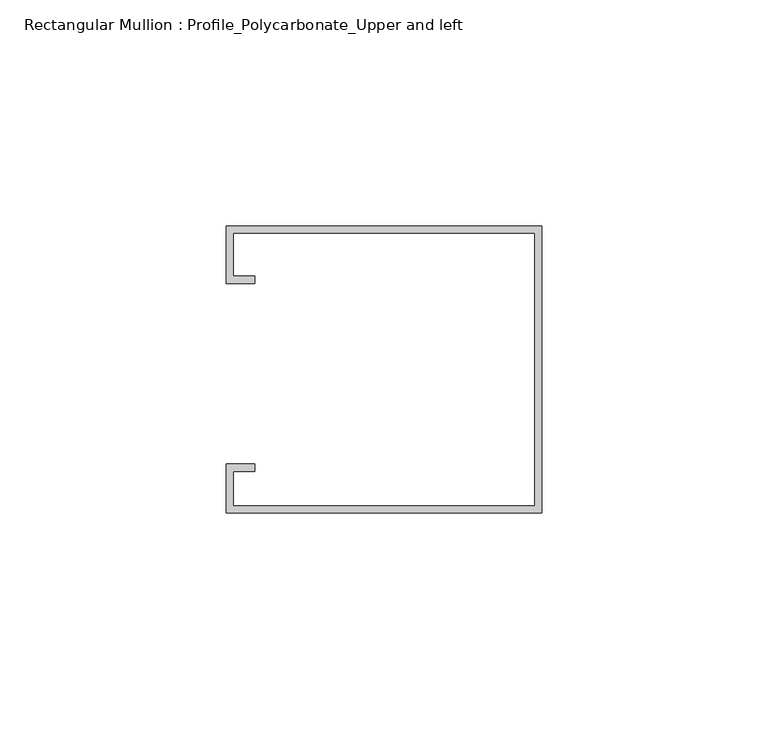
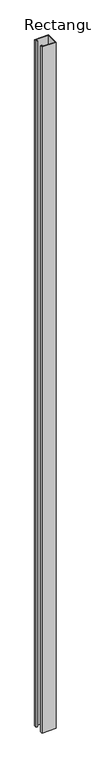
"""IFC4 building model written with IfcOpenShell, lengths in millimetres: member geometry, Rectangular Mullion : Profile_Polycarbonate_Upper and left."""

from ifc_helpers import new_model, si_unit, frame, origin, place, context, project, spatial, polyline, outline, extrude, source, transform, mapped, element, save


def rectangular_mullion_profile_polycarbonate_upper_and_left_59ea335d(model_context):
    return source(origin(), model_context, "Body", "SweptSolid", [
        extrude(outline(polyline([(0.0, 32.7), (0.0, -30.8), (-69.85, -30.8), (-69.85, -20.0), (-63.5, -20.0), (-63.5, -21.5875), (-68.2625, -21.5875), (-68.2625, -29.2125), (-1.5875, -29.2125), (-1.5875, 31.1125), (-68.2625, 31.1125), (-68.2625, 21.5875), (-63.5, 21.5875), (-63.5, 20.0), (-69.85, 20.0), (-69.85, 32.7), (0.0, 32.7)])), frame((0.0, 0.0, -3644.8931569), z_axis=(0.0, 0.0, 1.0), x_axis=(1.0, 0.0, 0.0)), (0.0, 0.0, 1.0), 3644.8931569),
    ])


if __name__ == "__main__":
    model = new_model("IFC4")
    model_context = context("Model", 3, world=origin())
    ifc_project = project(units=[si_unit("LENGTHUNIT", "METRE", prefix="MILLI")], contexts=[model_context])
    site = spatial("IfcSite", under=ifc_project)
    building = spatial("IfcBuilding", under=site)
    placement = place(None, origin())
    rectangular_mullion_profile_polycarbonate_upper_and_left_shape = rectangular_mullion_profile_polycarbonate_upper_and_left_59ea335d(model_context)
    element("IfcMember", 1, ObjectType="Rectangular Mullion : Profile_Polycarbonate_Upper and left", at=placement, inside=building, context=model_context, shape_type="MappedRepresentation", body=[
        mapped(rectangular_mullion_profile_polycarbonate_upper_and_left_shape, transform((0.0, 0.0, 0.0), x_axis=(1.0, 0.0, 0.0), y_axis=(0.0, 1.0, 0.0), z_axis=(0.0, 0.0, 1.0))),
    ])
    save(model, "model.ifc")

# Revit data of these elements
# Type "Rectangular Mullion : Profile_Polycarbonate_Upper and left"
#   built-in parameter 1007322 = 0.208333 (stored number, unit not read)
#   built-in parameter 1007321 = 0.00520833 (stored number, unit not read)
#   built-in parameter 1007320 = 0 (stored number, unit not read)
